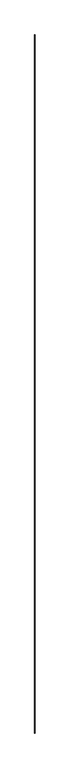
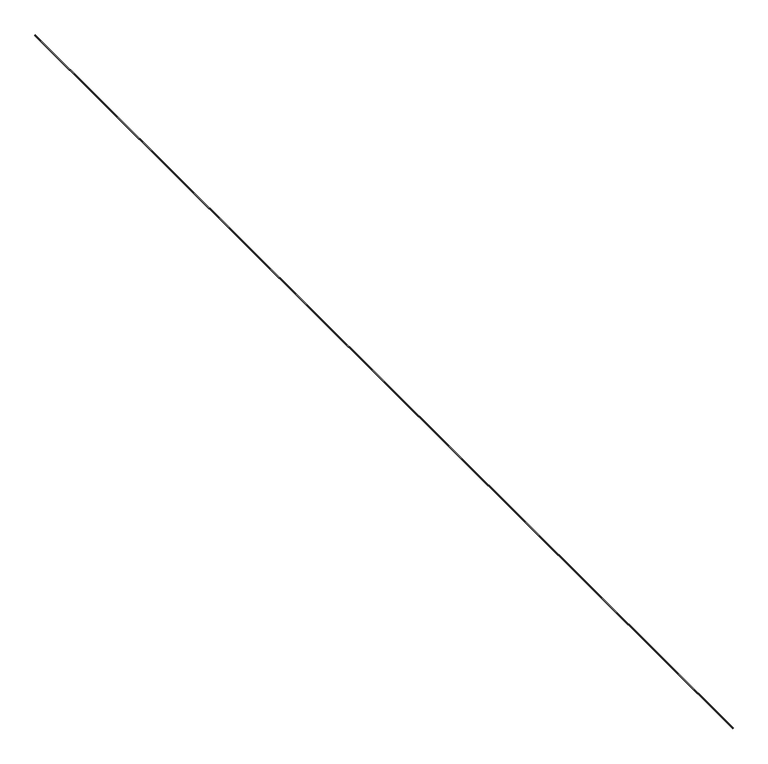
"""IFC4 building model written with IfcOpenShell, lengths in millimetres: proxy geometry, Inner panel:Inner panel:1:Inner panel:1 : Inner panel:Inner panel:300324:2:Inner panel:1:Inner panel:1 : Inner panel:Inner panel:300324:2 : Inner panel:Inner panel:1:Inner panel:1 : Inner panel:Inner panel:300324:300043:57 : Inner panel:Inner panel:1:Inner panel:1 : Inner panel:Inner panel:300324:2:Inner panel:1:Inner panel:1 : Inner panel:Inner panel:300324:2 : Inner panel:Inner panel:1:Inner panel:1 : Inner panel:Inner panel:300324:300043:308120."""

from ifc_helpers import new_model, si_unit, frame, origin, place, context, project, spatial, polyline, outline, extrude, source, transform, mapped, element, save


def generic_models_5554b964(model_context):
    return source(origin(), model_context, "Body", "SweptSolid", [
        extrude(outline(polyline([(3849.5738455, 558873.0669745), (3851.1599693, 558911.1339445), (3889.2269394, 558909.5478208), (3887.6408156, 558871.4808507), (3849.5738455, 558873.0669745)]), holes=[polyline([(3852.0521639, 558875.3470274), (3885.3607627, 558873.9591691), (3886.748621, 558907.2677679), (3853.4400222, 558908.6556262), (3852.0521639, 558875.3470274)])]), frame((0.0, -579346.5018006, 0.0), z_axis=(0.0, 1.0, 0.0), x_axis=(0.0, 0.0, 1.0)), (0.0, 0.0, 1.0), 88442.8),
    ])


if __name__ == "__main__":
    model = new_model("IFC4")
    model_context = context("Model", 3, world=origin())
    ifc_project = project(units=[si_unit("LENGTHUNIT", "METRE", prefix="MILLI")], contexts=[model_context])
    site = spatial("IfcSite", under=ifc_project)
    building = spatial("IfcBuilding", under=site)
    placement = place(None, origin())
    generic_models_shape = generic_models_5554b964(model_context)
    element("IfcBuildingElementProxy", 1, Name="Inner panel:Inner panel:1:Inner panel:1 : Inner panel:Inner panel:300324:2:Inner panel:1:Inner panel:1 : Inner panel:Inner panel:300324:2 : Inner panel:Inner panel:1:Inner panel:1 : Inner panel:Inner panel:300324:300043:57 : Inner panel:Inner panel:1:Inner panel:1 : Inner panel:Inner panel:300324:2:Inner panel:1:Inner panel:1 : Inner panel:Inner panel:300324:2 : Inner panel:Inner panel:1:Inner panel:1 : Inner panel:Inner panel:300324:300043:308120", ObjectType="Inner panel:Inner panel:1:Inner panel:1 : Inner panel:Inner panel:300324:2:Inner panel:1:Inner panel:1 : Inner panel:Inner panel:300324:2 : Inner panel:Inner panel:1:Inner panel:1 : Inner panel:Inner panel:300324:300043:57 : Inner panel:Inner panel:1:Inner panel:1 : Inner panel:Inner panel:300324:2:Inner panel:1:Inner panel:1 : Inner panel:Inner panel:300324:2 : Inner panel:Inner panel:1:Inner panel:1 : Inner panel:Inner panel:300324:300043:308120", at=placement, inside=building, context=model_context, shape_type="MappedRepresentation", body=[
        mapped(generic_models_shape, transform((0.0, 0.0, 0.0), x_axis=(1.0, 0.0, 0.0), y_axis=(0.0, 1.0, 0.0), z_axis=(0.0, 0.0, 1.0))),
    ])
    save(model, "model.ifc")

# Revit data of these elements
# Type "Inner panel:Inner panel:1:Inner panel:1 : Inner panel:Inner panel:300324:2:Inner panel:1:Inner panel:1 : Inner panel:Inner panel:300324:2 : Inner panel:Inner panel:1:Inner panel:1 : Inner panel:Inner panel:300324:300043:57 : Inner panel:Inner panel:1:Inner panel:1 : Inner panel:Inner panel:300324:2:Inner panel:1:Inner panel:1 : Inner panel:Inner panel:300324:2 : Inner panel:Inner panel:1:Inner panel:1 : Inner panel:Inner panel:300324:300043:308120"
#   NameOverride = "Inner panel:Inner panel:1:Inner panel:1 : Inner panel:Inner panel:300324:2:Inner panel:1:Inner panel:1 : Inner panel:Inner panel:300324:2 : Inner panel:Inner panel:1:Inner panel:1 : Inner panel:Inner panel:300324:300043:308120"
#   ObjectTypeOverride = "Inner panel:1:Inner panel:1 : Inner panel:Inner panel:300324:2 : Inner panel:Inner panel:1:Inner panel:1 : Inner panel:Inner panel:300324:300043"
#   Reference = "Inner panel"
#   Tag = "308120"
# Element 1 (IfcBuildingElementProxy, "Inner panel:Inner panel:1:Inner panel:1 : Inner panel:Inner panel:300324:2:Inner panel:1:Inner panel:1 : Inner panel:Inner panel:300324:2 : Inner panel:Inner panel:1:Inner panel:1 : Inner panel:Inner panel:300324:300043:57 : Inner panel:Inner panel:1:Inner panel:1 : Inner panel:Inner panel:300324:2:Inner panel:1:Inner panel:1 : Inner panel:Inner panel:300324:2 : Inner panel:Inner panel:1:Inner panel:1 : Inner panel:Inner panel:300324:300043:308120")
#   Materials on its faces: "1 1/2\" X 1 1/2\" x 1/8\" ALUM. TUBE (6061-T6) - (2) #16 WOOD SCREWS WITH 2.5\" EMBED AT EACH GLULAM - (1) SCREW AT ENDS"
# Materials
#   "1 1/2\" X 1 1/2\" x 1/8\" ALUM. TUBE (6061-T6) - (2) #16 WOOD SCREWS WITH 2.5\" EMBED AT EACH GLULAM - (1) SCREW AT ENDS": class "Unassigned", colour RGB 202 201 200, transparency 0, Cost = 0
